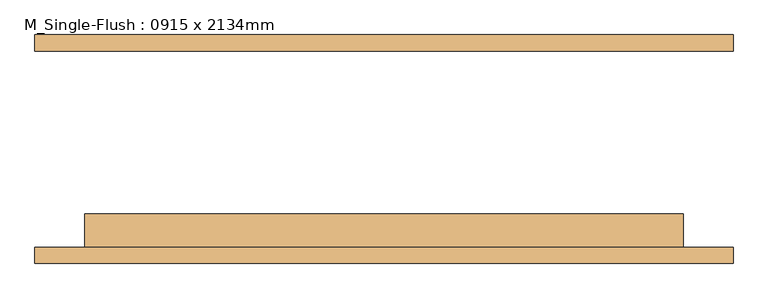
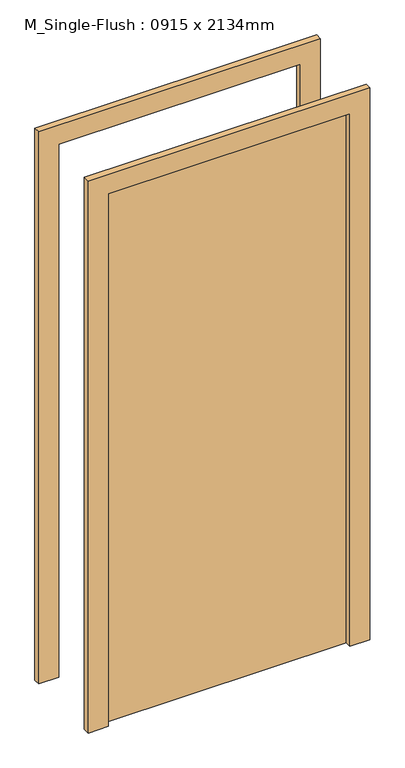
"""IFC4 building model written with IfcOpenShell, lengths in millimetres: door geometry, M_Single-Flush : 0915 x 2134mm."""

from ifc_helpers import new_model, si_unit, frame, origin, origin_with_axes, place, context, project, spatial, polyline, outline, extrude, source, transform, mapped, element, save


def m_single_flush_0915_x_2134mm_1c84716f(model_context):
    return source(origin(), model_context, "Body", "SweptSolid", [
        extrude(outline(polyline([(2210.0, -533.5), (0.0, -533.5), (0.0, -457.5), (2134.0, -457.5), (2134.0, 457.5), (0.0, 457.5), (0.0, 533.5), (2210.0, 533.5), (2210.0, -533.5)])), frame((0.0, -175.0, 0.0), z_axis=(0.0, 1.0, 0.0), x_axis=(0.0, 0.0, 1.0)), (0.0, 0.0, 1.0), 25.0),
        extrude(outline(polyline([(2210.0, 533.5), (2210.0, -533.5), (0.0, -533.5), (0.0, -457.5), (2134.0, -457.5), (2134.0, 457.5), (0.0, 457.5), (0.0, 533.5), (2210.0, 533.5)])), frame((0.0, 150.0, 0.0), z_axis=(0.0, 1.0, 0.0), x_axis=(0.0, 0.0, 1.0)), (0.0, 0.0, 1.0), 25.0),
        extrude(outline(polyline([(457.5, -99.0), (457.5, -150.0), (-457.5, -150.0), (-457.5, -99.0), (457.5, -99.0)])), origin_with_axes(), (0.0, 0.0, 1.0), 2134.0),
    ])


if __name__ == "__main__":
    model = new_model("IFC4")
    model_context = context("Model", 3, world=origin())
    ifc_project = project(units=[si_unit("LENGTHUNIT", "METRE", prefix="MILLI")], contexts=[model_context])
    site = spatial("IfcSite", under=ifc_project)
    building = spatial("IfcBuilding", under=site)
    placement = place(None, origin())
    m_single_flush_0915_x_2134mm_shape = m_single_flush_0915_x_2134mm_1c84716f(model_context)
    element("IfcDoor", 1, ObjectType="M_Single-Flush : 0915 x 2134mm", at=placement, inside=building, context=model_context, shape_type="MappedRepresentation", body=[
        mapped(m_single_flush_0915_x_2134mm_shape, transform((0.0, 0.0, 0.0), x_axis=(1.0, 0.0, 0.0), y_axis=(0.0, 1.0, 0.0), z_axis=(0.0, 0.0, 1.0))),
    ])
    save(model, "model.ifc")

# Revit data of these elements
# Type "M_Single-Flush : 0915 x 2134mm"
#   Type Mark = "20"
#   Thickness = 0.051 m
#   Height = 2.134 m
#   Trim Projection Ext = 0.025 m
#   Trim Projection Int = 0.025 m
#   Trim Width = 0.076 m
#   Width = 0.915 m
#   Door Material = Door - Panel
#   Frame Material = Door - Frame
#   Function = (empty or 0)
#   Wall Closure = (empty or 0)
# Element 1 (IfcDoor, "M_Single-Flush : 0915 x 2134mm")
#   Materials on its faces: "Door - Frame", "Door - Panel"
# Materials
#   "Door - Panel": class "Wood", colour RGB 210 159 95, transparency 0
#   "Door - Frame": class "Miscellaneous", colour RGB 118 70 51, transparency 0
